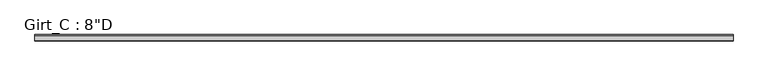
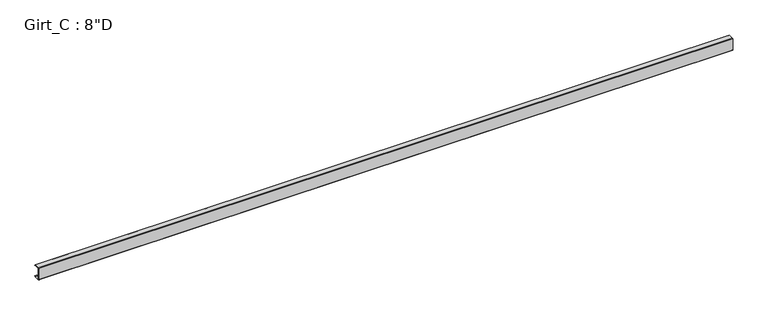
"""IFC4 building model written with IfcOpenShell, lengths in millimetres: beam geometry."""

from ifc_helpers import new_model, si_unit, point, frame, frame_2d, origin, place, context, project, spatial, polyline, circle_curve, trimmed, segment, composite_curve, outline, extrude, source, transform, mapped, element, save


def beam_0ee53da3(model_context):
    return source(origin(), model_context, "Body", "SweptSolid", [
        extrude(outline(composite_curve([segment(polyline([(87.5109375, 101.6), (99.7560415, 87.0068534), (97.6278742, 85.221109), (86.2154765, 98.821875), (3.3005807, 98.821875)]), True, "CONTINUOUS"), segment(trimmed(circle_curve(frame_2d((3.3741066, 96.8381931)), 1.9850441), [point((3.3005807, 98.821875))], [point((1.3890625, 96.8381931))], True, "CARTESIAN"), True, "CONTINUOUS"), segment(polyline([(1.3890625, 96.8381931), (1.3890625, -96.8389339)]), True, "CONTINUOUS"), segment(trimmed(circle_curve(frame_2d((3.3748024, -96.8389339)), 1.9857399), [point((1.3890625, -96.8389339))], [point((3.2694106, -98.821875))], True, "CARTESIAN"), True, "CONTINUOUS"), segment(polyline([(3.2694106, -98.821875), (86.2154765, -98.821875), (97.6510975, -85.1934327), (99.7792647, -86.979177), (87.5109375, -101.6), (3.3734375, -101.6)]), True, "CONTINUOUS"), segment(trimmed(circle_curve(frame_2d((3.3734375, -96.8375)), 4.7625), [point((3.3734375, -101.6))], [point((-1.3890625, -96.8375))], False, "CARTESIAN"), True, "CONTINUOUS"), segment(polyline([(-1.3890625, -96.8375), (-1.3890625, 96.8375)]), True, "CONTINUOUS"), segment(trimmed(circle_curve(frame_2d((3.3734375, 96.8375)), 4.7625), [point((-1.3890625, 96.8375))], [point((3.3734375, 101.6))], False, "CARTESIAN"), True, "CONTINUOUS"), segment(polyline([(3.3734375, 101.6), (87.5109375, 101.6)]), True, "CONTINUOUS")], self_intersect=False)), frame((-5564.0649169, 0.0, 0.0), z_axis=(1.0, 0.0, 0.0), x_axis=(0.0, 1.0, 0.0)), (0.0, 0.0, 1.0), 11128.1298339),
    ])


if __name__ == "__main__":
    model = new_model("IFC4")
    model_context = context("Model", 3, world=origin())
    ifc_project = project(units=[si_unit("LENGTHUNIT", "METRE", prefix="MILLI")], contexts=[model_context])
    site = spatial("IfcSite", under=ifc_project)
    building = spatial("IfcBuilding", under=site)
    placement = place(None, origin())
    beam_shape = beam_0ee53da3(model_context)
    element("IfcBeam", 1, ObjectType="Girt_C : 8\"D", at=placement, inside=building, context=model_context, shape_type="MappedRepresentation", body=[
        mapped(beam_shape, transform((0.0, 0.0, 0.0), x_axis=(1.0, 0.0, 0.0), y_axis=(0.0, 1.0, 0.0), z_axis=(0.0, 0.0, 1.0))),
    ])
    save(model, "model.ifc")

# Revit data of these elements
# Type "Girt_C : 8\"D"
#   half leg = 0' - 1 3/4"
#   Web_Thickness = 0' - 0 7/64"
#   Length [instance default] = 10' - 0"
#   Leg_1 = 0' - 3 1/2"
#   Height = 0' - 8"
#   Structural Material [instance default] = none
# Element 1 (IfcBeam, "Girt_C : 8\"D")
#   Structural Material = GALVANIZED 'CEE' SECTION (8.0x3.5C - SEE STRUCT. DWGS)
#   Materials on its faces: "GALVANIZED 'CEE' SECTION (8.0x3.5C - SEE STRUCT. DWGS)"
# Materials
#   "GALVANIZED 'CEE' SECTION (8.0x3.5C - SEE STRUCT. DWGS)": class "Metal", colour RGB 137 146 153, transparency 0, Description = "Steel, mill finish", Cost = 0
